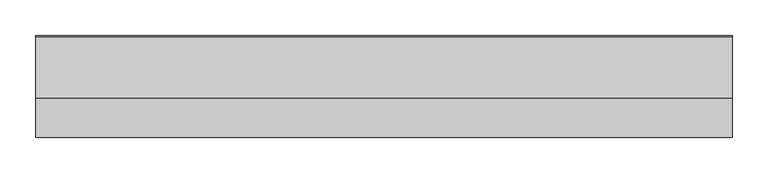
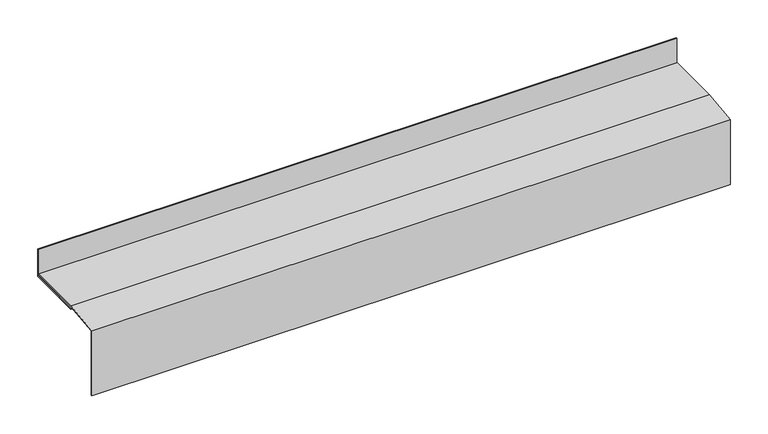
"""IFC4 building model written with IfcOpenShell, lengths in millimetres: proxy geometry, Generic Models 7:Generic Models 1:7:Generic Models 1:7 : Generic Models 7:Generic Models 1:337419:4 : Generic Models 7:Generic Models 1:7:Generic Models 1:7 : Generic Models 7:Generic Models 1:337419:315055."""

from ifc_helpers import new_model, si_unit, origin, place, context, project, spatial, faceted_brep, source, transform, mapped, element, save


def generic_models_aa1b3fda(model_context):
    return source(origin(), model_context, "Body", "Brep", [
        faceted_brep([(593738.0867239, -579143.2285706, -81.7582633), (593738.0867239, -579143.2285706, 22.8699913), (593738.0867239, -579089.2994022, 28.8582208), (593738.0867239, -579003.8194128, 28.8582208), (593738.0867239, -579003.8194128, 30.4457208), (593738.0867239, -579089.3872692, 30.4457208), (593738.0867239, -579144.8160706, 24.2909738), (593738.0867239, -579144.8160706, -81.7582633), (592758.9138536, -579143.2285706, -81.7582633), (592758.9138536, -579143.2285706, 22.8699913), (592758.9138536, -579144.8160706, 24.2909738), (592758.9138536, -579144.8160706, -81.7582633), (592758.9138536, -579089.2994022, 28.8582208), (592758.9138536, -579056.8670584, 28.8582208), (592758.9138536, -579003.8194128, 28.8582208), (592758.9138536, -579003.8194128, 30.4457208), (592758.9138536, -579058.4545584, 30.4457208), (592758.9138536, -579089.3872692, 30.4457208)], [[[0, 1, 2, 3, 4, 5, 6, 7]], [[1, 0, 8, 9]], [[7, 6, 10, 11]], [[0, 7, 11, 8]], [[2, 1, 9, 12]], [[3, 2, 12, 13, 14]], [[4, 3, 14, 15]], [[5, 4, 15, 16, 17]], [[6, 5, 17, 10]], [[8, 11, 10, 17, 16, 15, 14, 13, 12, 9]]]),
        faceted_brep([(592758.9138536, -579002.9968291, 27.0981204), (592758.9138536, -579002.9968291, 69.9933987), (592758.9138536, -579001.4093291, 69.9933987), (592758.9138536, -579001.4093291, 25.5106204), (592758.9138536, -579089.5913841, 25.5106204), (592758.9138536, -579089.5913841, 27.0981204), (593738.0867239, -579089.5913841, 27.0981204), (593738.0867239, -579002.9968291, 27.0981204), (593738.0867239, -579089.5913841, 25.5106204), (593738.0867239, -579001.4093291, 25.5106204), (593738.0867239, -579001.4093291, 69.9933987), (593738.0867239, -579002.9968291, 69.9933987)], [[[0, 1, 2, 3, 4, 5]], [[6, 7, 0, 5]], [[8, 6, 5, 4]], [[9, 8, 4, 3]], [[10, 9, 3, 2]], [[11, 10, 2, 1]], [[7, 11, 1, 0]], [[7, 6, 8, 9, 10, 11]]]),
    ])


if __name__ == "__main__":
    model = new_model("IFC4")
    model_context = context("Model", 3, world=origin())
    ifc_project = project(units=[si_unit("LENGTHUNIT", "METRE", prefix="MILLI")], contexts=[model_context])
    site = spatial("IfcSite", under=ifc_project)
    building = spatial("IfcBuilding", under=site)
    placement = place(None, origin())
    generic_models_shape = generic_models_aa1b3fda(model_context)
    element("IfcBuildingElementProxy", 1, Name="Generic Models 7:Generic Models 1:7:Generic Models 1:7 : Generic Models 7:Generic Models 1:337419:4 : Generic Models 7:Generic Models 1:7:Generic Models 1:7 : Generic Models 7:Generic Models 1:337419:315055", ObjectType="Generic Models 7:Generic Models 1:7:Generic Models 1:7 : Generic Models 7:Generic Models 1:337419:4 : Generic Models 7:Generic Models 1:7:Generic Models 1:7 : Generic Models 7:Generic Models 1:337419:315055", at=placement, inside=building, context=model_context, shape_type="MappedRepresentation", body=[
        mapped(generic_models_shape, transform((0.0, 0.0, 0.0), x_axis=(1.0, 0.0, 0.0), y_axis=(0.0, 1.0, 0.0), z_axis=(0.0, 0.0, 1.0))),
    ])
    save(model, "model.ifc")

# Revit data of these elements
# Type "Generic Models 7:Generic Models 1:7:Generic Models 1:7 : Generic Models 7:Generic Models 1:337419:4 : Generic Models 7:Generic Models 1:7:Generic Models 1:7 : Generic Models 7:Generic Models 1:337419:315055"
#   NameOverride = "Generic Models 7:Generic Models 1:7:Generic Models 1:7 : Generic Models 7:Generic Models 1:337419:315055"
#   ObjectTypeOverride = "Generic Models 1:7 : Generic Models 7:Generic Models 1:337419"
#   Reference = "Generic Models 1"
#   Tag = "315055"
# Element 1 (IfcBuildingElementProxy, "Generic Models 7:Generic Models 1:7:Generic Models 1:7 : Generic Models 7:Generic Models 1:337419:4 : Generic Models 7:Generic Models 1:7:Generic Models 1:7 : Generic Models 7:Generic Models 1:337419:315055")
#   Materials on its faces: "ANODIZED ALUM. FLASHING - MATCH STOREFRONT (ALIGN WITH OTHER WALL ASSEMBLIES)"
# Materials
#   "ANODIZED ALUM. FLASHING - MATCH STOREFRONT (ALIGN WITH OTHER WALL ASSEMBLIES)": class "Unassigned", colour RGB 210 209 208, transparency 0, Cost = 0
